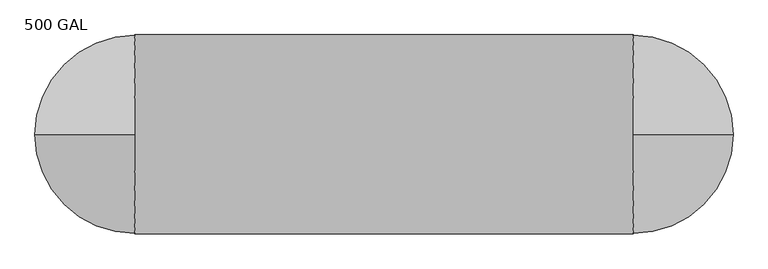
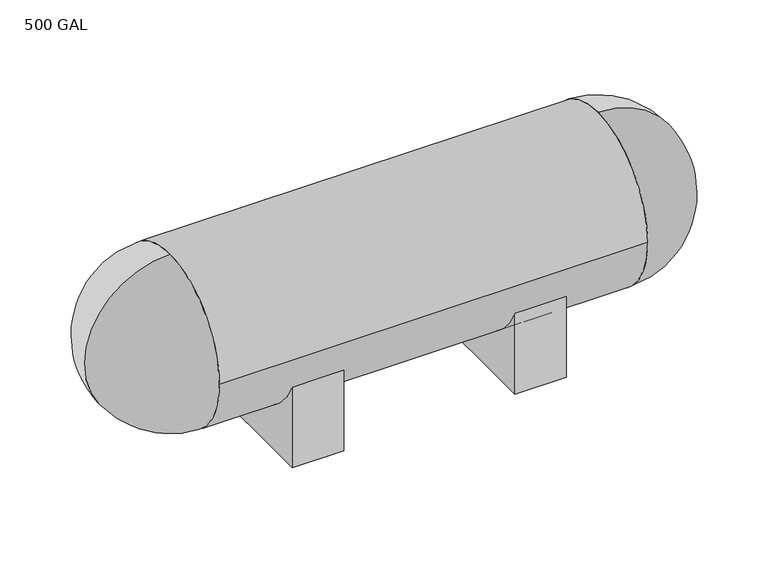
"""IFC4 building model written with IfcOpenShell, lengths in millimetres: geographic element geometry, LPG Tanks - Above Surface (AUS) : 500 GAL."""

from ifc_helpers import new_model, si_unit, point, frame, frame_2d, origin, place, context, project, spatial, polyline, circle_curve, ellipse_curve, trimmed, segment, composite_curve, outline, extrude, source, transform, mapped, element, save
from ifc_brep_helpers import plane_surface, revolved_surface, advanced_brep


def geographic_element_500_gal_7660307d(model_context):
    return source(origin(), model_context, "Body", "SolidModel", [
        advanced_brep(
        [(-949.6208556, 0.0, 355.6), (-695.6208556, 0.0, 609.6), (-695.6208556, 0.0, 101.6), (-695.6208556, 0.0, 355.6)],
        [
            (0, 1, circle_curve(frame((-695.6208556, 0.0, 355.6), z_axis=(0.0, 1.0, 0.0), x_axis=(1.0, 0.0, 0.0)), 254.0)),
            (1, 2, circle_curve(frame((-695.6208556, 0.0, 355.6), z_axis=(-1.0, 0.0, 0.0), x_axis=(0.0, 0.0, 1.0)), 254.0)),
            (2, 0, circle_curve(frame((-695.6208556, 0.0, 355.6), z_axis=(0.0, 1.0, 0.0), x_axis=(1.0, 0.0, 0.0)), 254.0)),
            (2, 1, circle_curve(frame((-695.6208556, 0.0, 355.6), z_axis=(-1.0, 0.0, 0.0), x_axis=(0.0, 0.0, 1.0)), 254.0)),
            (1, 3),
            (3, 2),
        ],
        [
            revolved_surface(trimmed(ellipse_curve(frame((-695.6208556, 0.0, 355.6), z_axis=(0.0, -1.0, 0.0), x_axis=(1.0, 0.0, 0.0)), 254.0, 254.0), [point((-695.6208556, 0.0, 609.6))], [point((-949.6208556, 0.0, 355.6))], True, "CARTESIAN"), (-1089.3208556, 0.0, 355.6), (-1.0, 0.0, 0.0)),
            plane_surface(frame((-695.6208556, 0.0, 355.6), z_axis=(1.0, 0.0, 0.0), x_axis=(0.0, 0.0, 1.0))),
        ],
        [
            (0, [[1, 2, 3]]),
            (0, [[-3, 4, -1]]),
            (1, [[-2, 5, 6]]),
            (1, [[-4, -6, -5]]),
        ],
    ),
        advanced_brep(
        [(574.3791444, 0.0, 101.6), (574.3791444, 0.0, 609.6), (828.3791444, 0.0, 355.6), (574.3791444, 0.0, 355.6)],
        [
            (0, 1, circle_curve(frame((574.3791444, 0.0, 355.6), z_axis=(1.0, 0.0, 0.0), x_axis=(0.0, 0.0, 1.0)), 254.0)),
            (1, 2, circle_curve(frame((574.3791444, 0.0, 355.6), z_axis=(0.0, 1.0, 0.0), x_axis=(1.0, 0.0, 0.0)), 254.0)),
            (2, 0, circle_curve(frame((574.3791444, 0.0, 355.6), z_axis=(0.0, 1.0, 0.0), x_axis=(1.0, 0.0, 0.0)), 254.0)),
            (1, 0, circle_curve(frame((574.3791444, 0.0, 355.6), z_axis=(1.0, 0.0, 0.0), x_axis=(0.0, 0.0, 1.0)), 254.0)),
            (3, 1),
            (0, 3),
        ],
        [
            revolved_surface(trimmed(ellipse_curve(frame((574.3791444, 0.0, 355.6), z_axis=(0.0, -1.0, 0.0), x_axis=(1.0, 0.0, 0.0)), 254.0, 254.0), [point((828.3791444, 0.0, 355.6))], [point((574.3791444, 0.0, 609.6))], True, "CARTESIAN"), (167.9791444, 0.0, 355.6), (-1.0, 0.0, 0.0)),
            plane_surface(frame((574.3791444, 0.0, 355.6), z_axis=(-1.0, 0.0, 0.0), x_axis=(0.0, 0.0, 1.0))),
        ],
        [
            (0, [[1, 2, 3]]),
            (0, [[4, -3, -2]]),
            (1, [[5, -1, 6]]),
            (1, [[-6, -4, -5]]),
        ],
    ),
        extrude(outline(composite_curve([segment(trimmed(circle_curve(frame_2d((0.0, 355.6)), 254.0), [point((-254.0, 355.6))], [point((254.0, 355.6))], False, "CARTESIAN"), True, "CONTINUOUS"), segment(trimmed(circle_curve(frame_2d((0.0, 355.6)), 254.0), [point((254.0, 355.6))], [point((-254.0, 355.6))], False, "CARTESIAN"), True, "CONTINUOUS")], self_intersect=False)), frame((-695.6208556, 0.0, 0.0), z_axis=(1.0, 0.0, 0.0), x_axis=(0.0, 1.0, 0.0)), (0.0, 0.0, 1.0), 1270.0),
        extrude(outline(composite_curve([segment(polyline([(232.7948453, 0.0), (-232.7948453, 0.0), (-232.7948453, 254.0)]), True, "CONTINUOUS"), segment(trimmed(circle_curve(frame_2d((0.0, 355.6)), 254.0), [point((-232.7948453, 254.0))], [point((232.7948453, 254.0))], True, "CARTESIAN"), True, "CONTINUOUS"), segment(polyline([(232.7948453, 254.0), (232.7948453, 0.0)]), True, "CONTINUOUS")], self_intersect=False)), frame((193.3791444, 0.0, 0.0), z_axis=(1.0, 0.0, 0.0), x_axis=(0.0, 1.0, 0.0)), (0.0, 0.0, 1.0), 152.4),
        extrude(outline(composite_curve([segment(polyline([(232.7948453, 0.0), (-232.7948453, 0.0), (-232.7948453, 254.0)]), True, "CONTINUOUS"), segment(trimmed(circle_curve(frame_2d((0.0, 355.6)), 254.0), [point((-232.7948453, 254.0))], [point((232.7948453, 254.0))], True, "CARTESIAN"), True, "CONTINUOUS"), segment(polyline([(232.7948453, 254.0), (232.7948453, 0.0)]), True, "CONTINUOUS")], self_intersect=False)), frame((-467.0208556, 0.0, 0.0), z_axis=(1.0, 0.0, 0.0), x_axis=(0.0, 1.0, 0.0)), (0.0, 0.0, 1.0), 152.4),
    ])


if __name__ == "__main__":
    model = new_model("IFC4")
    model_context = context("Model", 3, world=origin())
    ifc_project = project(units=[si_unit("LENGTHUNIT", "METRE", prefix="MILLI")], contexts=[model_context])
    site = spatial("IfcSite", under=ifc_project)
    building = spatial("IfcBuilding", under=site)
    placement = place(None, origin())
    geographic_element_500_gal_shape = geographic_element_500_gal_7660307d(model_context)
    element("IfcGeographicElement", 1, ObjectType="LPG Tanks - Above Surface (AUS) : 500 GAL", at=placement, inside=building, context=model_context, shape_type="MappedRepresentation", body=[
        mapped(geographic_element_500_gal_shape, transform((0.0, 0.0, 0.0), x_axis=(1.0, 0.0, 0.0), y_axis=(0.0, 1.0, 0.0), z_axis=(0.0, 0.0, 1.0))),
    ])
    save(model, "model.ifc")

# Revit data of these elements
# Type "LPG Tanks - Above Surface (AUS) : 500 GAL"
#   COBie.Type.CreatedBy = "design@eagle.com"
#   COBie.Type.CreatedOn = "2016-10-27T05:31:12"
#   COBie.Type.Name = "LPG Tanks - Above Surface (AUS)_500 GAL"
#   COBie.Type.Category = "G30"
#   COBie.Type.Description = "LPG Tanks - Above Surface (AUS)_500 GAL"
#   COBie.Type.Manufacturer = ""
#   COBie.Type.ModelNumber = ""
#   Assembly Code = "G30"
#   COBie.Type.ReplacementCost = 0
#   DIAMETER = 1' - 8"
#   HEIGHT = 0' - 4"
#   HEIGHT AFF - CENTER = 1' - 2"
#   LEGS OFFSET = 1' - 0"
#   MINIMUM CLEARANCE FROM BUILDING = 10' - 0"
#   TANK RADIUS = 0' - 10"
#   TANK WIDTH = 5' - 10"
#   WIDTH = 4' - 2"
#   COBie.Type = yes
# Element 1 (IfcGeographicElement, "LPG Tanks - Above Surface (AUS) : 500 GAL")
#   Materials on its faces: "01 - LPG TANKS"
# Materials
#   "01 - LPG TANKS": class "Miscellaneous", colour RGB 127 127 127, transparency 0
